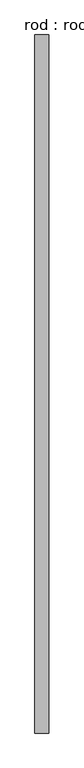
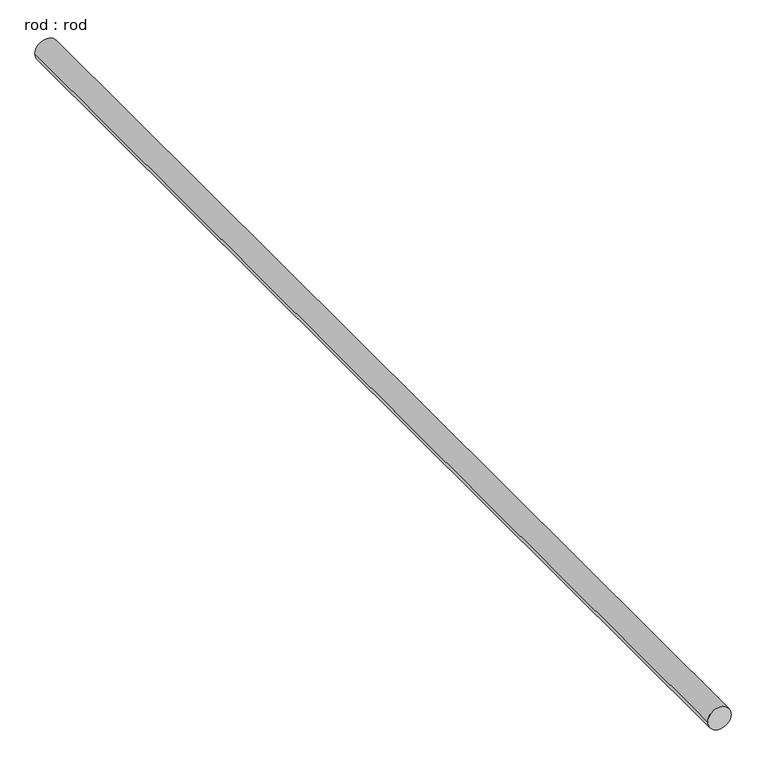
"""IFC4 building model written with IfcOpenShell, lengths in millimetres: proxy geometry, rod : rod."""

from ifc_helpers import new_model, si_unit, point, frame, frame_2d, origin, place, context, project, spatial, circle_curve, trimmed, segment, composite_curve, outline, extrude, source, transform, mapped, element, save


def rod_rod_72a6f481(model_context):
    return source(origin(), model_context, "Body", "SweptSolid", [
        extrude(outline(composite_curve([segment(trimmed(circle_curve(frame_2d((0.0108462, 0.0)), 200.0), [point((0.0108462, 200.0))], [point((0.0108462, -200.0))], False, "CARTESIAN"), True, "CONTINUOUS"), segment(trimmed(circle_curve(frame_2d((0.0108462, 0.0)), 200.0), [point((0.0108462, -200.0))], [point((0.0108462, 200.0))], False, "CARTESIAN"), True, "CONTINUOUS")], self_intersect=False)), frame((0.0, -5876.902337, 0.0), z_axis=(0.0, 1.0, 0.0), x_axis=(0.0, 0.0, 1.0)), (0.0, 0.0, 1.0), 19939.2619047),
    ])


if __name__ == "__main__":
    model = new_model("IFC4")
    model_context = context("Model", 3, world=origin())
    ifc_project = project(units=[si_unit("LENGTHUNIT", "METRE", prefix="MILLI")], contexts=[model_context])
    site = spatial("IfcSite", under=ifc_project)
    building = spatial("IfcBuilding", under=site)
    placement = place(None, origin())
    rod_rod_shape = rod_rod_72a6f481(model_context)
    element("IfcBuildingElementProxy", 1, Name="rod : rod", ObjectType="rod : rod", at=placement, inside=building, context=model_context, shape_type="MappedRepresentation", body=[
        mapped(rod_rod_shape, transform((0.0, 0.0, 0.0), x_axis=(1.0, 0.0, 0.0), y_axis=(0.0, 1.0, 0.0), z_axis=(0.0, 0.0, 1.0))),
    ])
    save(model, "model.ifc")

# Revit data of these elements
# Type "rod : rod"
#   Default Elevation = 0
